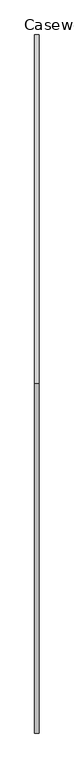
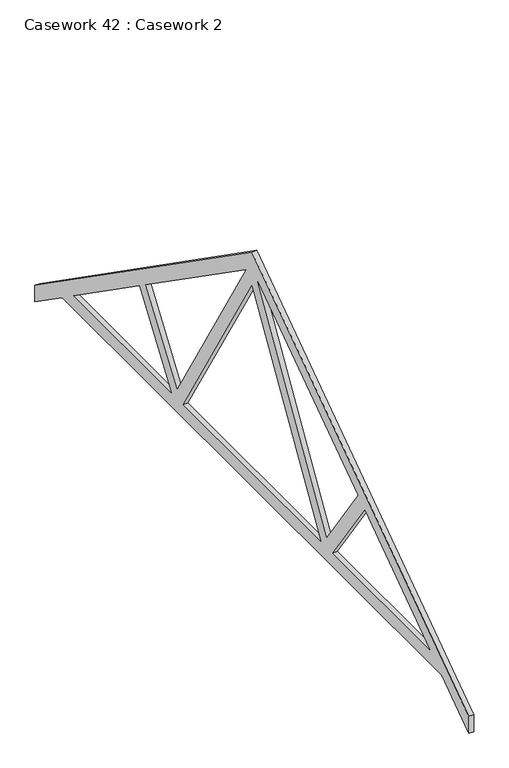
"""IFC4 building model written with IfcOpenShell, lengths in millimetres: furniture geometry, Casework 42 : Casework 2."""

from ifc_helpers import new_model, si_unit, frame, origin, place, context, project, spatial, polyline, outline, extrude, source, transform, mapped, element, save


def casework_42_casework_2_e9decabd(model_context):
    return source(origin(), model_context, "Body", "SweptSolid", [
        extrude(outline(polyline([(6583.1149316, 5252.5), (-277.3850684, 5252.5), (-767.3850684, 4909.3983063), (-767.3850684, 5092.5144946), (3152.8649316, 7837.5030963), (7073.1149316, 5092.5144946), (7073.1149316, 4909.3983063), (6583.1149316, 5252.5)]), holes=[polyline([(4612.3149663, 5402.5), (6368.8927306, 5402.5), (5190.2113591, 6227.8215815), (4612.3149663, 5402.5)]), polyline([(4394.2037684, 5402.5), (3152.8649316, 7468.4347567), (1911.5260948, 5402.5), (4394.2037684, 5402.5)]), polyline([(4504.5438357, 5510.1038939), (5067.3385525, 6313.8580469), (3262.0771677, 7577.915677), (4504.5438357, 5510.1038939)]), polyline([(1693.4148969, 5402.5), (1115.5185041, 6227.8215815), (-63.1628674, 5402.5), (1693.4148969, 5402.5)]), polyline([(1801.1860276, 5510.1038939), (3043.6526956, 7577.915677), (1238.3913108, 6313.8580469), (1801.1860276, 5510.1038939)])]), frame((-8021.5247381, 0.0, 0.0), z_axis=(1.0, 0.0, 0.0), x_axis=(0.0, 1.0, 0.0)), (0.0, 0.0, 1.0), 49.6351915),
    ])


if __name__ == "__main__":
    model = new_model("IFC4")
    model_context = context("Model", 3, world=origin())
    ifc_project = project(units=[si_unit("LENGTHUNIT", "METRE", prefix="MILLI")], contexts=[model_context])
    site = spatial("IfcSite", under=ifc_project)
    building = spatial("IfcBuilding", under=site)
    placement = place(None, origin())
    casework_42_casework_2_shape = casework_42_casework_2_e9decabd(model_context)
    element("IfcFurniture", 1, ObjectType="Casework 42 : Casework 2", at=placement, inside=building, context=model_context, shape_type="MappedRepresentation", body=[
        mapped(casework_42_casework_2_shape, transform((0.0, 0.0, 0.0), x_axis=(1.0, 0.0, 0.0), y_axis=(0.0, 1.0, 0.0), z_axis=(0.0, 0.0, 1.0))),
    ])
    save(model, "model.ifc")

# Revit data of these elements
# Element 1 (IfcFurniture, "Casework 42 : Casework 2")
#   Materials on its faces: "Softwood, Lumber"
# Materials
#   "Softwood, Lumber": class "Wood", colour RGB 205 156 65, transparency 0, Description = "Pinus Echinata", Cost = 0
